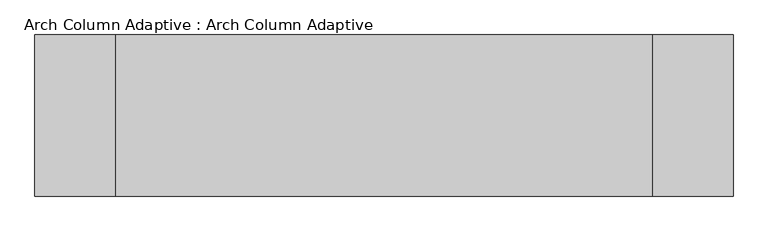
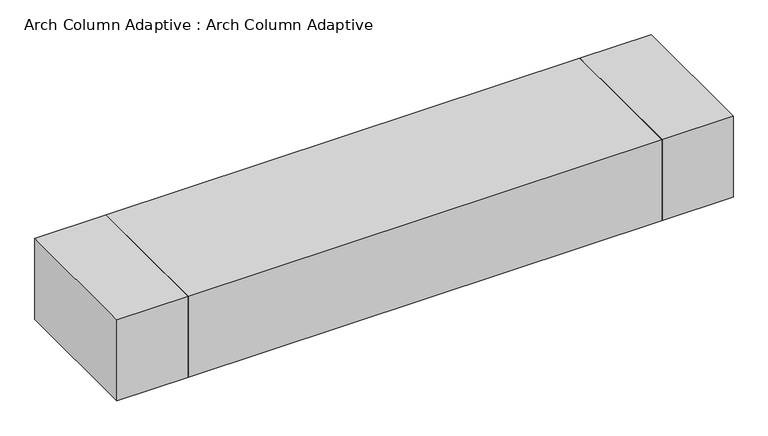
"""IFC4 building model written with IfcOpenShell, lengths in millimetres: proxy geometry, Arch Column Adaptive : Arch Column Adaptive."""

from ifc_helpers import new_model, si_unit, frame, origin, place, context, project, spatial, polyline, outline, extrude, source, transform, mapped, element, save


def arch_column_adaptive_arch_column_adaptive_b670a59b(model_context):
    return source(origin(), model_context, "Body", "SweptSolid", [
        extrude(outline(polyline([(5000.0, -1500.0), (5000.0, 1500.0), (6500.0, 1500.0), (6500.0, -1500.0), (5000.0, -1500.0)])), frame((0.0, 0.0, 21310.0), z_axis=(0.0, 0.0, 1.0), x_axis=(1.0, 0.0, 0.0)), (0.0, 0.0, 1.0), 1800.0),
        extrude(outline(polyline([(-5000.0, 1500.0), (-5000.0, -1500.0), (-6500.0, -1500.0), (-6500.0, 1500.0), (-5000.0, 1500.0)])), frame((0.0, 0.0, 21310.0), z_axis=(0.0, 0.0, 1.0), x_axis=(1.0, 0.0, 0.0)), (0.0, 0.0, 1.0), 1800.0),
        extrude(outline(polyline([(-5000.0, -1500.0), (-5000.0, 1500.0), (5000.0, 1500.0), (5000.0, -1500.0), (-5000.0, -1500.0)])), frame((0.0, 0.0, 21310.0), z_axis=(0.0, 0.0, 1.0), x_axis=(1.0, 0.0, 0.0)), (0.0, 0.0, 1.0), 1800.0),
    ])


if __name__ == "__main__":
    model = new_model("IFC4")
    model_context = context("Model", 3, world=origin())
    ifc_project = project(units=[si_unit("LENGTHUNIT", "METRE", prefix="MILLI")], contexts=[model_context])
    site = spatial("IfcSite", under=ifc_project)
    building = spatial("IfcBuilding", under=site)
    placement = place(None, origin())
    arch_column_adaptive_arch_column_adaptive_shape = arch_column_adaptive_arch_column_adaptive_b670a59b(model_context)
    element("IfcBuildingElementProxy", 1, Name="Arch Column Adaptive : Arch Column Adaptive", ObjectType="Arch Column Adaptive : Arch Column Adaptive", at=placement, inside=building, context=model_context, shape_type="MappedRepresentation", body=[
        mapped(arch_column_adaptive_arch_column_adaptive_shape, transform((0.0, 0.0, 0.0), x_axis=(1.0, 0.0, 0.0), y_axis=(0.0, 1.0, 0.0), z_axis=(0.0, 0.0, 1.0))),
    ])
    save(model, "model.ifc")

# Revit data of these elements
# Type "Arch Column Adaptive : Arch Column Adaptive"
#   Top Width = 3000 mm
#   Length [instance default] = 21000 mm
#   Height [instance default] = 50000 mm
#   Default Elevation = 0
# Element 1 (IfcBuildingElementProxy, "Arch Column Adaptive : Arch Column Adaptive")
#   Height = 21310 mm
